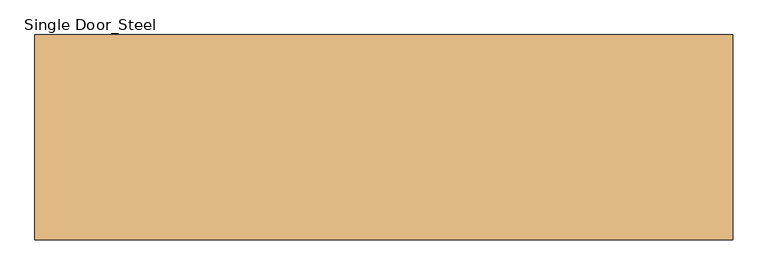
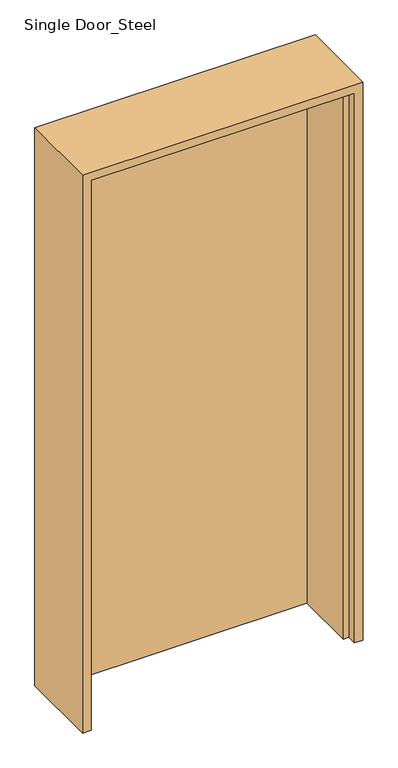
"""IFC4 building model written with IfcOpenShell, lengths in millimetres: door geometry, Single Door_Steel : H_DR_AMB_Single Door_Steel_W1000xH2100."""

from ifc_helpers import new_model, si_unit, origin, origin_with_axes, place, context, project, spatial, polyline, outline, extrude, faceted_brep, source, transform, mapped, element, save


def single_door_steel_aae97da1(model_context):
    return source(origin(), model_context, "Body", "SolidModel", [
        extrude(outline(polyline([(470.0, 147.0), (470.0, 112.0), (-470.0, 112.0), (-470.0, 147.0), (470.0, 147.0)])), origin_with_axes(), (0.0, 0.0, 1.0), 2070.0),
        faceted_brep([(470.0, 147.0, 0.0), (500.0, 147.0, 0.0), (500.0, -147.0, 0.0), (470.0, -147.0, 0.0), (470.0, -112.0, 0.0), (450.0, -112.0, 0.0), (450.0, 112.0, 0.0), (470.0, 112.0, 0.0), (470.0, 147.0, 2070.0), (-470.0, 147.0, 2070.0), (-470.0, 147.0, 0.0), (-500.0, 147.0, 0.0), (-500.0, 147.0, 2100.0), (500.0, 147.0, 2100.0), (500.0, -147.0, 2100.0), (-500.0, -147.0, 2100.0), (-500.0, -147.0, 0.0), (-470.0, -147.0, 0.0), (-470.0, -147.0, 2070.0), (470.0, -147.0, 2070.0), (470.0, -112.0, 2070.0), (-470.0, -112.0, 2070.0), (-470.0, -112.0, 0.0), (-450.0, -112.0, 0.0), (-450.0, -112.0, 2050.0), (450.0, -112.0, 2050.0), (450.0, 112.0, 2050.0), (-450.0, 112.0, 2050.0), (-450.0, 112.0, 0.0), (-470.0, 112.0, 0.0), (-470.0, 112.0, 2070.0), (470.0, 112.0, 2070.0)], [[[0, 1, 2, 3, 4, 5, 6, 7]], [[1, 0, 8, 9, 10, 11, 12, 13]], [[2, 1, 13, 14]], [[3, 2, 14, 15, 16, 17, 18, 19]], [[4, 3, 19, 20]], [[5, 4, 20, 21, 22, 23, 24, 25]], [[6, 5, 25, 26]], [[7, 6, 26, 27, 28, 29, 30, 31]], [[0, 7, 31, 8]], [[9, 30, 29, 10]], [[10, 29, 28, 23, 22, 17, 16, 11]], [[15, 12, 11, 16]], [[21, 18, 17, 22]], [[27, 24, 23, 28]], [[14, 13, 12, 15]], [[20, 19, 18, 21]], [[26, 25, 24, 27]], [[8, 31, 30, 9]]]),
    ])


if __name__ == "__main__":
    model = new_model("IFC4")
    model_context = context("Model", 3, world=origin())
    ifc_project = project(units=[si_unit("LENGTHUNIT", "METRE", prefix="MILLI")], contexts=[model_context])
    site = spatial("IfcSite", under=ifc_project)
    building = spatial("IfcBuilding", under=site)
    placement = place(None, origin())
    single_door_steel_shape = single_door_steel_aae97da1(model_context)
    element("IfcDoor", 1, ObjectType="Single Door_Steel : H_DR_AMB_Single Door_Steel_W1000xH2100", at=placement, inside=building, context=model_context, shape_type="MappedRepresentation", body=[
        mapped(single_door_steel_shape, transform((0.0, 0.0, 0.0), x_axis=(1.0, 0.0, 0.0), y_axis=(0.0, 1.0, 0.0), z_axis=(0.0, 0.0, 1.0))),
    ])
    save(model, "model.ifc")

# Revit data of these elements
# Type "Single Door_Steel : H_DR_AMB_Single Door_Steel_W1000xH2100"
#   Type Mark = "SD"
#   Analytic Construction = "<None>"
#   프레임 투영 외부. = 25 mm
#   프레임 투영 내부. = 25 mm
#   프레임 폭 = 75 mm
#   Height = 2100 mm
#   Width = 1000 mm
#   Define Thermal Properties by = 1
#   문 패널 = none
#   문 프레임 = none
#   Function = (empty or 0)
#   Wall Closure = (empty or 0)
